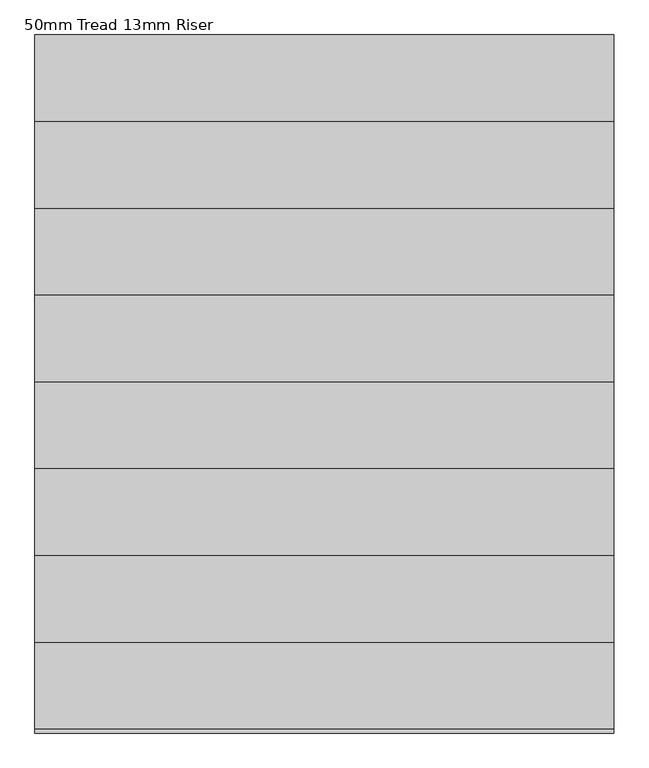
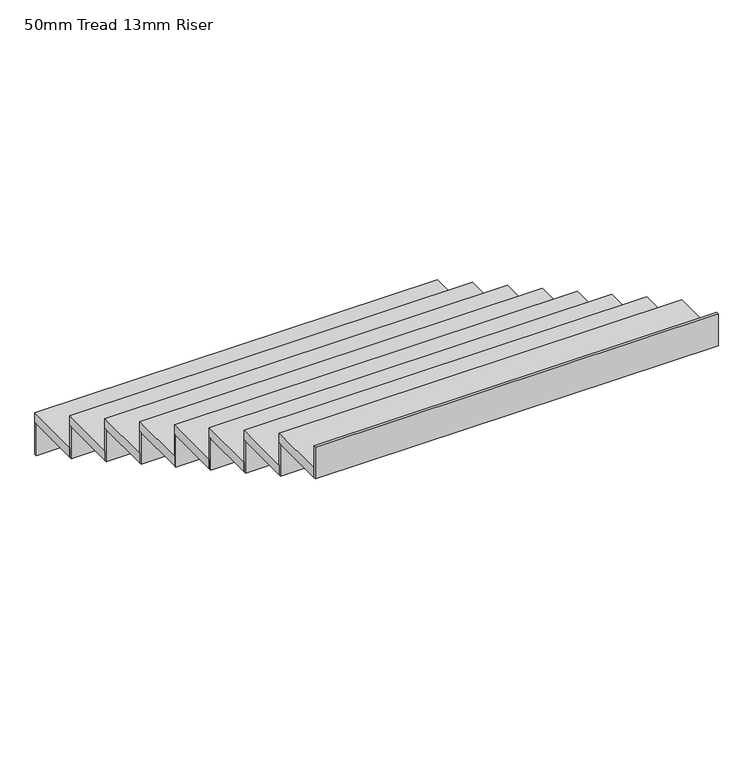
"""IFC4 building model written with IfcOpenShell, lengths in millimetres: stair flight geometry, 50mm Tread 13mm Riser."""

from ifc_helpers import new_model, si_unit, frame, origin, place, context, project, spatial, polyline, outline, extrude, source, transform, mapped, element, save


def stair_flight_50mm_tread_13mm_riser_277c3fa9(model_context):
    return source(origin(), model_context, "Body", "SweptSolid", [
        extrude(outline(polyline([(15000.0002442, 23517.4999999), (15000.0002442, 23529.9999999), (17000.0002442, 23529.9999999), (17000.0002442, 23517.4999999), (15000.0002442, 23517.4999999)])), frame((0.0, 0.0, 24950.0), z_axis=(0.0, 0.0, 1.0), x_axis=(1.0, 0.0, 0.0)), (0.0, 0.0, 1.0), 166.6666667),
        extrude(outline(polyline([(17000.0002442, 23229.9999999), (15000.0002442, 23229.9999999), (15000.0002442, 23529.9999999), (17000.0002442, 23529.9999999), (17000.0002442, 23229.9999999)])), frame((0.0, 0.0, 25116.6666667), z_axis=(0.0, 0.0, 1.0), x_axis=(1.0, 0.0, 0.0)), (0.0, 0.0, 1.0), 50.0),
        extrude(outline(polyline([(15000.0002442, 23217.4999999), (15000.0002442, 23229.9999999), (17000.0002442, 23229.9999999), (17000.0002442, 23217.4999999), (15000.0002442, 23217.4999999)])), frame((0.0, 0.0, 25116.6666667), z_axis=(0.0, 0.0, 1.0), x_axis=(1.0, 0.0, 0.0)), (0.0, 0.0, 1.0), 166.6666667),
        extrude(outline(polyline([(17000.0002442, 22929.9999999), (15000.0002442, 22929.9999999), (15000.0002442, 23229.9999999), (17000.0002442, 23229.9999999), (17000.0002442, 22929.9999999)])), frame((0.0, 0.0, 25283.3333333), z_axis=(0.0, 0.0, 1.0), x_axis=(1.0, 0.0, 0.0)), (0.0, 0.0, 1.0), 50.0),
        extrude(outline(polyline([(15000.0002442, 22917.4999999), (15000.0002442, 22929.9999999), (17000.0002442, 22929.9999999), (17000.0002442, 22917.4999999), (15000.0002442, 22917.4999999)])), frame((0.0, 0.0, 25283.3333333), z_axis=(0.0, 0.0, 1.0), x_axis=(1.0, 0.0, 0.0)), (0.0, 0.0, 1.0), 166.6666667),
        extrude(outline(polyline([(17000.0002442, 22629.9999999), (15000.0002442, 22629.9999999), (15000.0002442, 22929.9999999), (17000.0002442, 22929.9999999), (17000.0002442, 22629.9999999)])), frame((0.0, 0.0, 25450.0), z_axis=(0.0, 0.0, 1.0), x_axis=(1.0, 0.0, 0.0)), (0.0, 0.0, 1.0), 50.0),
        extrude(outline(polyline([(15000.0002442, 22617.4999999), (15000.0002442, 22629.9999999), (17000.0002442, 22629.9999999), (17000.0002442, 22617.4999999), (15000.0002442, 22617.4999999)])), frame((0.0, 0.0, 25450.0), z_axis=(0.0, 0.0, 1.0), x_axis=(1.0, 0.0, 0.0)), (0.0, 0.0, 1.0), 166.6666667),
        extrude(outline(polyline([(17000.0002442, 22329.9999999), (15000.0002442, 22329.9999999), (15000.0002442, 22629.9999999), (17000.0002442, 22629.9999999), (17000.0002442, 22329.9999999)])), frame((0.0, 0.0, 25616.6666667), z_axis=(0.0, 0.0, 1.0), x_axis=(1.0, 0.0, 0.0)), (0.0, 0.0, 1.0), 50.0),
        extrude(outline(polyline([(15000.0002442, 22317.4999999), (15000.0002442, 22329.9999999), (17000.0002442, 22329.9999999), (17000.0002442, 22317.4999999), (15000.0002442, 22317.4999999)])), frame((0.0, 0.0, 25616.6666667), z_axis=(0.0, 0.0, 1.0), x_axis=(1.0, 0.0, 0.0)), (0.0, 0.0, 1.0), 166.6666667),
        extrude(outline(polyline([(17000.0002442, 22029.9999999), (15000.0002442, 22029.9999999), (15000.0002442, 22329.9999999), (17000.0002442, 22329.9999999), (17000.0002442, 22029.9999999)])), frame((0.0, 0.0, 25783.3333333), z_axis=(0.0, 0.0, 1.0), x_axis=(1.0, 0.0, 0.0)), (0.0, 0.0, 1.0), 50.0),
        extrude(outline(polyline([(15000.0002442, 22017.4999999), (15000.0002442, 22029.9999999), (17000.0002442, 22029.9999999), (17000.0002442, 22017.4999999), (15000.0002442, 22017.4999999)])), frame((0.0, 0.0, 25783.3333333), z_axis=(0.0, 0.0, 1.0), x_axis=(1.0, 0.0, 0.0)), (0.0, 0.0, 1.0), 166.6666667),
        extrude(outline(polyline([(17000.0002442, 21729.9999999), (15000.0002442, 21729.9999999), (15000.0002442, 22029.9999999), (17000.0002442, 22029.9999999), (17000.0002442, 21729.9999999)])), frame((0.0, 0.0, 25950.0), z_axis=(0.0, 0.0, 1.0), x_axis=(1.0, 0.0, 0.0)), (0.0, 0.0, 1.0), 50.0),
        extrude(outline(polyline([(15000.0002442, 21717.4999999), (15000.0002442, 21729.9999999), (17000.0002442, 21729.9999999), (17000.0002442, 21717.4999999), (15000.0002442, 21717.4999999)])), frame((0.0, 0.0, 25950.0), z_axis=(0.0, 0.0, 1.0), x_axis=(1.0, 0.0, 0.0)), (0.0, 0.0, 1.0), 166.6666667),
        extrude(outline(polyline([(17000.0002442, 21429.9999999), (15000.0002442, 21429.9999999), (15000.0002442, 21729.9999999), (17000.0002442, 21729.9999999), (17000.0002442, 21429.9999999)])), frame((0.0, 0.0, 26116.6666667), z_axis=(0.0, 0.0, 1.0), x_axis=(1.0, 0.0, 0.0)), (0.0, 0.0, 1.0), 50.0),
        extrude(outline(polyline([(15000.0002442, 21417.4999999), (15000.0002442, 21429.9999999), (17000.0002442, 21429.9999999), (17000.0002442, 21417.4999999), (15000.0002442, 21417.4999999)])), frame((0.0, 0.0, 26116.6666667), z_axis=(0.0, 0.0, 1.0), x_axis=(1.0, 0.0, 0.0)), (0.0, 0.0, 1.0), 166.6666667),
        extrude(outline(polyline([(15000.0002442, 21117.4999999), (15000.0002442, 21129.9999999), (17000.0002442, 21129.9999999), (17000.0002442, 21117.4999999), (15000.0002442, 21117.4999999)])), frame((0.0, 0.0, 26283.3333333), z_axis=(0.0, 0.0, 1.0), x_axis=(1.0, 0.0, 0.0)), (0.0, 0.0, 1.0), 166.6666667),
        extrude(outline(polyline([(17000.0002442, 21129.9999999), (15000.0002442, 21129.9999999), (15000.0002442, 21429.9999999), (17000.0002442, 21429.9999999), (17000.0002442, 21129.9999999)])), frame((0.0, 0.0, 26283.3333333), z_axis=(0.0, 0.0, 1.0), x_axis=(1.0, 0.0, 0.0)), (0.0, 0.0, 1.0), 50.0),
    ])


if __name__ == "__main__":
    model = new_model("IFC4")
    model_context = context("Model", 3, world=origin())
    ifc_project = project(units=[si_unit("LENGTHUNIT", "METRE", prefix="MILLI")], contexts=[model_context])
    site = spatial("IfcSite", under=ifc_project)
    building = spatial("IfcBuilding", under=site)
    placement = place(None, origin())
    stair_flight_50mm_tread_13mm_riser_shape = stair_flight_50mm_tread_13mm_riser_277c3fa9(model_context)
    element("IfcStairFlight", 1, ObjectType="50mm Tread 13mm Riser", at=placement, inside=building, context=model_context, shape_type="MappedRepresentation", body=[
        mapped(stair_flight_50mm_tread_13mm_riser_shape, transform((0.0, 0.0, 0.0), x_axis=(1.0, 0.0, 0.0), y_axis=(0.0, 1.0, 0.0), z_axis=(0.0, 0.0, 1.0))),
    ])
    save(model, "model.ifc")
